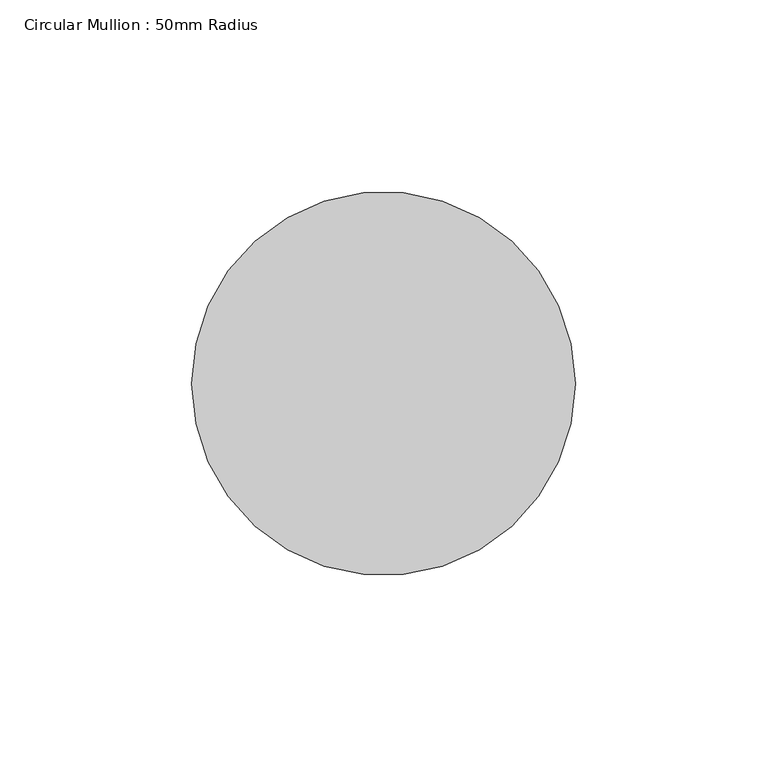
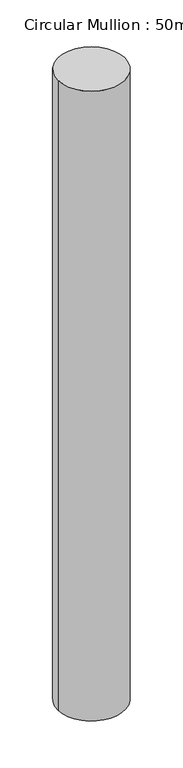
"""IFC4 building model written with IfcOpenShell, lengths in millimetres: member geometry, Circular Mullion : 50mm Radius."""

from ifc_helpers import new_model, si_unit, point, frame, origin, origin_2d, place, context, project, spatial, circle_curve, trimmed, segment, composite_curve, outline, extrude, source, transform, mapped, element, save


def circular_mullion_50mm_radius_5b1fa57e(model_context):
    return source(origin(), model_context, "Body", "SweptSolid", [
        extrude(outline(composite_curve([segment(trimmed(circle_curve(origin_2d(), 50.0), [point((50.0, 0.0))], [point((-50.0, 0.0))], False, "CARTESIAN"), True, "CONTINUOUS"), segment(trimmed(circle_curve(origin_2d(), 50.0), [point((-50.0, 0.0))], [point((50.0, 0.0))], False, "CARTESIAN"), True, "CONTINUOUS")], self_intersect=False)), frame((0.0, 0.0, -992.7871335), z_axis=(0.0, 0.0, 1.0), x_axis=(1.0, 0.0, 0.0)), (0.0, 0.0, 1.0), 992.7871335),
    ])


if __name__ == "__main__":
    model = new_model("IFC4")
    model_context = context("Model", 3, world=origin())
    ifc_project = project(units=[si_unit("LENGTHUNIT", "METRE", prefix="MILLI")], contexts=[model_context])
    site = spatial("IfcSite", under=ifc_project)
    building = spatial("IfcBuilding", under=site)
    placement = place(None, origin())
    circular_mullion_50mm_radius_shape = circular_mullion_50mm_radius_5b1fa57e(model_context)
    element("IfcMember", 1, ObjectType="Circular Mullion : 50mm Radius", at=placement, inside=building, context=model_context, shape_type="MappedRepresentation", body=[
        mapped(circular_mullion_50mm_radius_shape, transform((0.0, 0.0, 0.0), x_axis=(1.0, 0.0, 0.0), y_axis=(0.0, 1.0, 0.0), z_axis=(0.0, 0.0, 1.0))),
    ])
    save(model, "model.ifc")

# Revit data of these elements
# Type "Circular Mullion : 50mm Radius"
#   built-in parameter 1007350 = 0.164042 (stored number, unit not read)
# Element 1 (IfcMember, "Circular Mullion : 50mm Radius")
#   Materials on its faces: "Aluminium"
# Materials
#   "Aluminium": class "Metal", colour RGB 247 247 247, transparency 0, Description = "Aluminium 6061", Cost = 0
